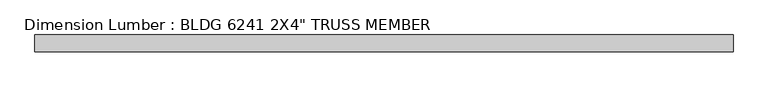
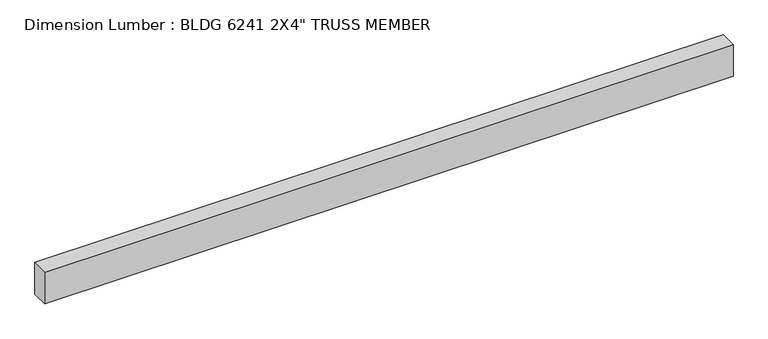
"""IFC4 building model written with IfcOpenShell, lengths in millimetres: beam geometry."""

from ifc_helpers import new_model, si_unit, frame, origin, place, context, project, spatial, polyline, outline, extrude, source, transform, mapped, element, save


def beam_b8261971(model_context):
    return source(origin(), model_context, "Body", "SweptSolid", [
        extrude(outline(polyline([(233.4866591, 25.4), (233.4866591, -25.4), (-1841.8619641, -25.4), (-1841.8619641, 25.4), (233.4866591, 25.4)])), frame((0.0, 0.0, -50.8), z_axis=(0.0, 0.0, 1.0), x_axis=(1.0, 0.0, 0.0)), (0.0, 0.0, 1.0), 101.6),
    ])


if __name__ == "__main__":
    model = new_model("IFC4")
    model_context = context("Model", 3, world=origin())
    ifc_project = project(units=[si_unit("LENGTHUNIT", "METRE", prefix="MILLI")], contexts=[model_context])
    site = spatial("IfcSite", under=ifc_project)
    building = spatial("IfcBuilding", under=site)
    placement = place(None, origin())
    beam_shape = beam_b8261971(model_context)
    element("IfcBeam", 1, ObjectType="Dimension Lumber : BLDG 6241 2X4\" TRUSS MEMBER", at=placement, inside=building, context=model_context, shape_type="MappedRepresentation", body=[
        mapped(beam_shape, transform((0.0, 0.0, 0.0), x_axis=(1.0, 0.0, 0.0), y_axis=(0.0, 1.0, 0.0), z_axis=(0.0, 0.0, 1.0))),
    ])
    save(model, "model.ifc")

# Revit data of these elements
# Type "Dimension Lumber : BLDG 6241 2X4\" TRUSS MEMBER"
#   Assembly Code = "B10"
#   A = 0.273472 SF
#   Length [instance default] = 5' - 0"
#   b = 0' - 2"
#   d = 0' - 4"
#   Structural Material [instance default] = Softwood, Lumber
# Element 1 (IfcBeam, "Dimension Lumber : BLDG 6241 2X4\" TRUSS MEMBER")
#   Materials on its faces: "Softwood, Lumber"
# Materials
#   "Softwood, Lumber": class "Wood", colour RGB 223 192 134, transparency 0, Description = "Pinus Echinata", Cost = 0
